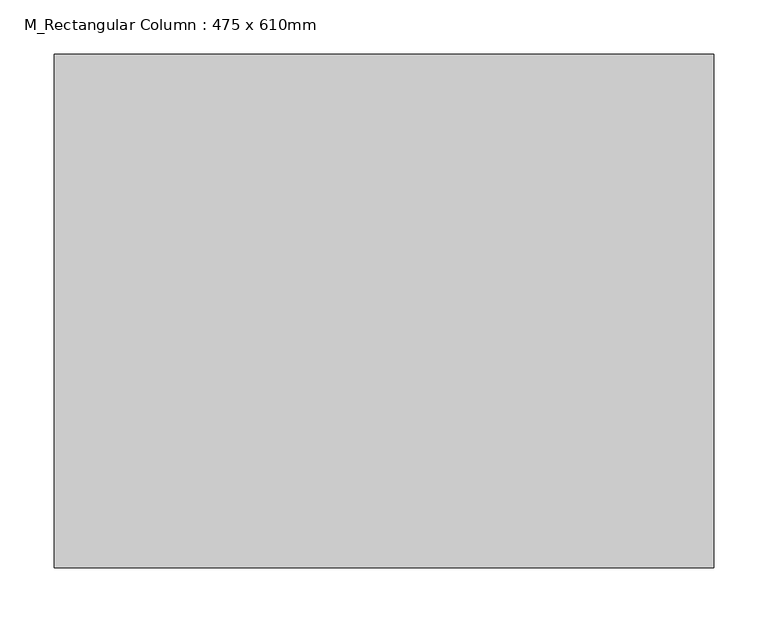
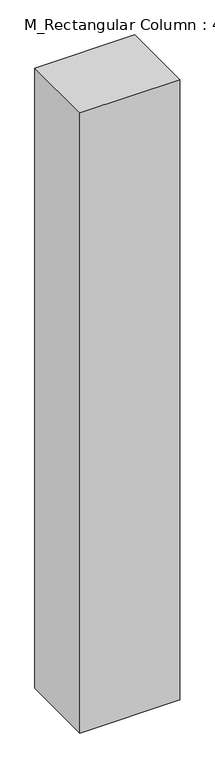
"""IFC4 building model written with IfcOpenShell, lengths in millimetres: column geometry, M_Rectangular Column : 475 x 610mm."""

from ifc_helpers import new_model, si_unit, frame, origin, place, context, project, spatial, polyline, outline, extrude, source, transform, mapped, element, save


def m_rectangular_column_475_x_610mm_e62a7db6(model_context):
    return source(origin(), model_context, "Body", "SweptSolid", [
        extrude(outline(polyline([(305.0, 237.5), (305.0, -237.5), (-305.0, -237.5), (-305.0, 237.5), (305.0, 237.5)])), frame((0.0, 0.0, 2000.0), z_axis=(0.0, 0.0, 1.0), x_axis=(1.0, 0.0, 0.0)), (0.0, 0.0, 1.0), 4000.0),
    ])


if __name__ == "__main__":
    model = new_model("IFC4")
    model_context = context("Model", 3, world=origin())
    ifc_project = project(units=[si_unit("LENGTHUNIT", "METRE", prefix="MILLI")], contexts=[model_context])
    site = spatial("IfcSite", under=ifc_project)
    building = spatial("IfcBuilding", under=site)
    placement = place(None, origin())
    m_rectangular_column_475_x_610mm_shape = m_rectangular_column_475_x_610mm_e62a7db6(model_context)
    element("IfcColumn", 1, ObjectType="M_Rectangular Column : 475 x 610mm", at=placement, inside=building, context=model_context, shape_type="MappedRepresentation", body=[
        mapped(m_rectangular_column_475_x_610mm_shape, transform((0.0, 0.0, 0.0), x_axis=(1.0, 0.0, 0.0), y_axis=(0.0, 1.0, 0.0), z_axis=(0.0, 0.0, 1.0))),
    ])
    save(model, "model.ifc")

# Revit data of these elements
# Type "M_Rectangular Column : 475 x 610mm"
#   Depth = 475 mm
#   Offset Base = 0 mm
#   Offset Top = 0 mm
#   Width = 610 mm
#   Material = Copper
# Element 1 (IfcColumn, "M_Rectangular Column : 475 x 610mm")
#   Materials on its faces: "Copper"
# Materials
#   "Copper": class "Metal", colour RGB 0 0 0, transparency 0, Description = "Copper, matte finish", Cost = 0
